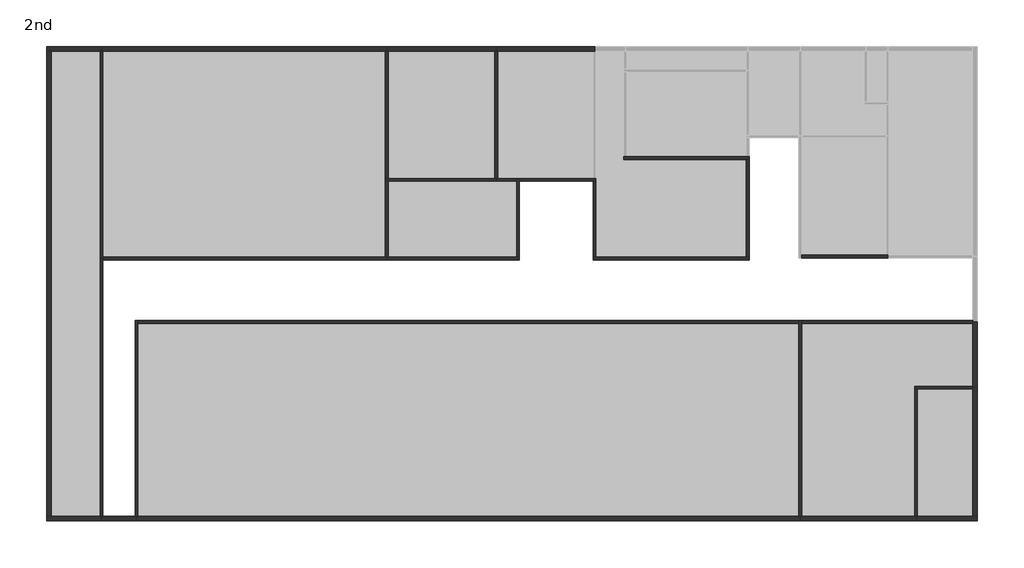
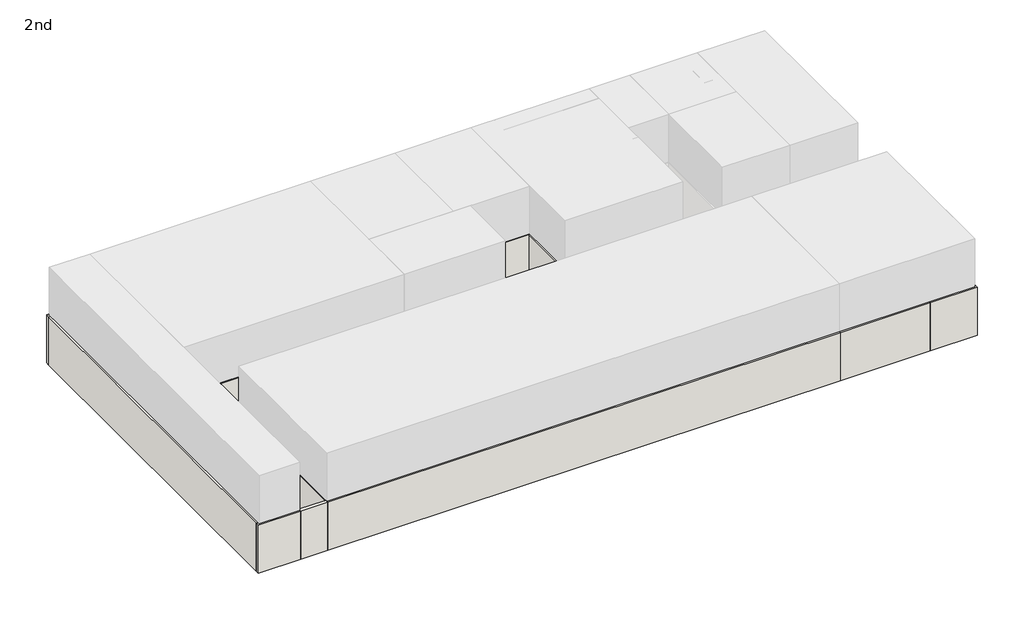
# One storey, part 1 of 2: 56 walls.
"""IFC4 building model written with IfcOpenShell, lengths in millimetres."""

from ifc_helpers import new_model, si_unit, frame, origin, place, context, project, spatial, polyline, outline, extrude, faceted_brep, element, save

model = new_model("IFC4")

# Units and contexts
model_context = context("Model", 3, world=origin())
ifc_project = project(units=[si_unit("LENGTHUNIT", "METRE", prefix="MILLI")], contexts=[model_context])

# Site, building, storey
site = spatial("IfcSite", under=ifc_project)
building = spatial("IfcBuilding", under=site)
storey = spatial("IfcBuildingStorey", under=building, Name="2nd", Elevation=14000.0)

# Walls
placement = place(None, origin())
element("IfcWall", 1, ObjectType="Wall-Ext_215Bwk", at=placement, inside=storey, context=model_context, shape_type="Brep", body=[
    faceted_brep([(11750.0, 151142.5, 14000.0), (42100.0, 151142.5, 14000.0), (42100.0, 151142.5, 17000.0), (11750.0, 151142.5, 17000.0), (11750.0, 151357.5, 14000.0), (11750.0, 151357.5, 17000.0), (11812.5, 151357.5, 17000.0), (42037.5, 151357.5, 17000.0), (42100.0, 151357.5, 17000.0), (42100.0, 151357.5, 14000.0), (42037.5, 151357.5, 14000.0), (11812.5, 151357.5, 14000.0)], [[[0, 1, 2, 3]], [[4, 5, 6, 7, 8, 9, 10, 11]], [[1, 0, 4, 11, 10, 9]], [[2, 1, 9, 8]], [[3, 2, 8, 7, 6, 5]], [[0, 3, 5, 4]]]),
])
element("IfcWall", 2, ObjectType="Wall-Ext_215Bwk", at=placement, inside=storey, context=model_context, shape_type="Brep", body=[
    faceted_brep([(23200.0, 172857.5, 14000.0), (10150.0, 172857.5, 14000.0), (10150.0, 172857.5, 17000.0), (23200.0, 172857.5, 17000.0), (23200.0, 172642.5, 14000.0), (23200.0, 172642.5, 17000.0), (23137.5, 172642.5, 17000.0), (10212.5, 172642.5, 17000.0), (10150.0, 172642.5, 17000.0), (10150.0, 172642.5, 14000.0), (10212.5, 172642.5, 14000.0), (23137.5, 172642.5, 14000.0)], [[[0, 1, 2, 3]], [[4, 5, 6, 7, 8, 9, 10, 11]], [[1, 0, 4, 11, 10, 9]], [[2, 1, 9, 8]], [[3, 2, 8, 7, 6, 5]], [[0, 3, 5, 4]]]),
])
element("IfcWall", 3, ObjectType="Wall-Ext_215Bwk", at=placement, inside=storey, context=model_context, shape_type="Brep", body=[
    faceted_brep([(28200.0, 172857.5, 14000.0), (23200.0, 172857.5, 14000.0), (23200.0, 172857.5, 17000.0), (28200.0, 172857.5, 17000.0), (28200.0, 172642.5, 14000.0), (28200.0, 172642.5, 17000.0), (28137.5, 172642.5, 17000.0), (23262.5, 172642.5, 17000.0), (23200.0, 172642.5, 17000.0), (23200.0, 172642.5, 14000.0), (23262.5, 172642.5, 14000.0), (28137.5, 172642.5, 14000.0)], [[[0, 1, 2, 3]], [[4, 5, 6, 7, 8, 9, 10, 11]], [[1, 0, 4, 11, 10, 9]], [[2, 1, 9, 8]], [[3, 2, 8, 7, 6, 5]], [[0, 3, 5, 4]]]),
])
element("IfcWall", 4, ObjectType="Wall-Ext_215Bwk", at=placement, inside=storey, context=model_context, shape_type="SweptSolid", body=[
    extrude(outline(polyline([(7642.5, 151357.5), (7642.5, 172642.5), (7857.5, 172642.5), (7857.5, 151357.5), (7642.5, 151357.5)])), frame((0.0, 0.0, 14000.0), z_axis=(0.0, 0.0, 1.0), x_axis=(1.0, 0.0, 0.0)), (0.0, 0.0, 1.0), 3000.0),
])
element("IfcWall", 5, ObjectType="Wall-Ext_215Bwk", at=placement, inside=storey, context=model_context, shape_type="Brep", body=[
    faceted_brep([(7642.5, 151142.5, 14000.0), (10150.0, 151142.5, 14000.0), (10150.0, 151142.5, 17000.0), (7642.5, 151142.5, 17000.0), (7642.5, 151357.5, 14000.0), (7642.5, 151357.5, 17000.0), (7857.5, 151357.5, 17000.0), (10087.5, 151357.5, 17000.0), (10150.0, 151357.5, 17000.0), (10150.0, 151357.5, 14000.0), (10087.5, 151357.5, 14000.0), (7857.5, 151357.5, 14000.0)], [[[0, 1, 2, 3]], [[4, 5, 6, 7, 8, 9, 10, 11]], [[1, 0, 4, 11, 10, 9]], [[2, 1, 9, 8]], [[3, 2, 8, 7, 6, 5]], [[0, 3, 5, 4]]]),
])
element("IfcWall", 6, ObjectType="Wall-Ext_215Bwk", at=placement, inside=storey, context=model_context, shape_type="Brep", body=[
    faceted_brep([(10150.0, 172857.5, 14000.0), (7642.5, 172857.5, 14000.0), (7642.5, 172857.5, 17000.0), (10150.0, 172857.5, 17000.0), (10150.0, 172642.5, 14000.0), (10150.0, 172642.5, 17000.0), (10087.5, 172642.5, 17000.0), (7857.5, 172642.5, 17000.0), (7642.5, 172642.5, 17000.0), (7642.5, 172642.5, 14000.0), (7857.5, 172642.5, 14000.0), (10087.5, 172642.5, 14000.0)], [[[0, 1, 2, 3]], [[4, 5, 6, 7, 8, 9, 10, 11]], [[1, 0, 4, 11, 10, 9]], [[3, 2, 8, 7, 6, 5]], [[0, 3, 5, 4]], [[2, 1, 9, 8]]]),
])
element("IfcWall", 7, ObjectType="Wall-Ext_215Bwk", at=placement, inside=storey, context=model_context, shape_type="Brep", body=[
    faceted_brep([(32700.0, 172857.5, 14000.0), (28200.0, 172857.5, 14000.0), (28200.0, 172857.5, 17000.0), (32700.0, 172857.5, 17000.0), (32700.0, 172642.5, 14000.0), (32700.0, 172642.5, 17000.0), (32637.5, 172642.5, 17000.0), (28262.5, 172642.5, 17000.0), (28200.0, 172642.5, 17000.0), (28200.0, 172642.5, 14000.0), (28262.5, 172642.5, 14000.0), (32637.5, 172642.5, 14000.0)], [[[0, 1, 2, 3]], [[4, 5, 6, 7, 8, 9, 10, 11]], [[1, 0, 4, 11, 10, 9]], [[2, 1, 9, 8]], [[3, 2, 8, 7, 6, 5]], [[0, 3, 5, 4]]]),
])
element("IfcWall", 8, ObjectType="Wall-Ext_215Bwk", at=placement, inside=storey, context=model_context, shape_type="Brep", body=[
    faceted_brep([(50207.5, 157250.0, 14000.0), (50207.5, 160250.0, 14000.0), (50207.5, 160250.0, 17000.0), (50207.5, 157250.0, 17000.0), (49992.5, 157250.0, 14000.0), (49992.5, 157250.0, 17000.0), (49992.5, 157312.5, 17000.0), (49992.5, 160187.5, 17000.0), (49992.5, 160250.0, 17000.0), (49992.5, 160250.0, 14000.0), (49992.5, 160187.5, 14000.0), (49992.5, 157312.5, 14000.0)], [[[0, 1, 2, 3]], [[4, 5, 6, 7, 8, 9, 10, 11]], [[1, 0, 4, 11, 10, 9]], [[2, 1, 9, 8]], [[3, 2, 8, 7, 6, 5]], [[0, 3, 5, 4]]]),
])
element("IfcWall", 9, ObjectType="Wall-Ext_215Bwk", at=placement, inside=storey, context=model_context, shape_type="Brep", body=[
    faceted_brep([(42100.0, 151142.5, 14000.0), (47400.0, 151142.5, 14000.0), (47400.0, 151142.5, 17000.0), (42100.0, 151142.5, 17000.0), (42100.0, 151357.5, 14000.0), (42100.0, 151357.5, 17000.0), (42162.5, 151357.5, 17000.0), (47337.5, 151357.5, 17000.0), (47400.0, 151357.5, 17000.0), (47400.0, 151357.5, 14000.0), (47337.5, 151357.5, 14000.0), (42162.5, 151357.5, 14000.0)], [[[0, 1, 2, 3]], [[4, 5, 6, 7, 8, 9, 10, 11]], [[1, 0, 4, 11, 10, 9]], [[2, 1, 9, 8]], [[3, 2, 8, 7, 6, 5]], [[0, 3, 5, 4]]]),
])
element("IfcWall", 10, ObjectType="Wall-Ext_215Bwk", at=placement, inside=storey, context=model_context, shape_type="Brep", body=[
    faceted_brep([(50207.5, 151357.5, 14000.0), (50207.5, 157250.0, 14000.0), (50207.5, 157250.0, 17000.0), (50207.5, 151357.5, 17000.0), (49992.5, 151357.5, 14000.0), (49992.5, 151357.5, 17000.0), (49992.5, 157187.5, 17000.0), (49992.5, 157250.0, 17000.0), (49992.5, 157250.0, 14000.0), (49992.5, 157187.5, 14000.0)], [[[0, 1, 2, 3]], [[4, 5, 6, 7, 8, 9]], [[1, 0, 4, 9, 8]], [[2, 1, 8, 7]], [[3, 2, 7, 6, 5]], [[0, 3, 5, 4]]]),
])
element("IfcWall", 11, ObjectType="Wall-Ext_215Bwk", at=placement, inside=storey, context=model_context, shape_type="Brep", body=[
    faceted_brep([(47400.0, 151142.5, 14000.0), (50207.5, 151142.5, 14000.0), (50207.5, 151142.5, 17000.0), (47400.0, 151142.5, 17000.0), (47400.0, 151357.5, 14000.0), (47400.0, 151357.5, 17000.0), (47462.5, 151357.5, 17000.0), (49992.5, 151357.5, 17000.0), (50207.5, 151357.5, 17000.0), (50207.5, 151357.5, 14000.0), (49992.5, 151357.5, 14000.0), (47462.5, 151357.5, 14000.0)], [[[0, 1, 2, 3]], [[4, 5, 6, 7, 8, 9, 10, 11]], [[1, 0, 4, 11, 10, 9]], [[3, 2, 8, 7, 6, 5]], [[0, 3, 5, 4]], [[2, 1, 9, 8]]]),
])
element("IfcWall", 12, ObjectType="Wall-Ext_215Bwk", at=placement, inside=storey, context=model_context, shape_type="Brep", body=[
    faceted_brep([(10150.0, 151142.5, 14000.0), (11750.0, 151142.5, 14000.0), (11750.0, 151142.5, 17000.0), (10150.0, 151142.5, 17000.0), (10150.0, 151357.5, 14000.0), (10150.0, 151357.5, 17000.0), (10212.5, 151357.5, 17000.0), (11687.5, 151357.5, 17000.0), (11750.0, 151357.5, 17000.0), (11750.0, 151357.5, 14000.0), (11687.5, 151357.5, 14000.0), (10212.5, 151357.5, 14000.0)], [[[0, 1, 2, 3]], [[4, 5, 6, 7, 8, 9, 10, 11]], [[1, 0, 4, 11, 10, 9]], [[2, 1, 9, 8]], [[3, 2, 8, 7, 6, 5]], [[0, 3, 5, 4]]]),
])
element("IfcWall", 13, ObjectType="Wall-Int_12P-100Blk-12P", at=placement, inside=storey, context=model_context, shape_type="SweptSolid", body=[
    extrude(outline(polyline([(11812.5, 160312.5), (42037.5, 160312.5), (42037.5, 160187.5), (11812.5, 160187.5), (11812.5, 160312.5)])), frame((0.0, 0.0, 14000.0), z_axis=(0.0, 0.0, 1.0), x_axis=(1.0, 0.0, 0.0)), (0.0, 0.0, 1.0), 3000.0),
])
element("IfcWall", 14, ObjectType="Wall-Int_12P-100Blk-12P", at=placement, inside=storey, context=model_context, shape_type="Brep", body=[
    faceted_brep([(11687.5, 160312.5, 14000.0), (11687.5, 151357.5, 14000.0), (11687.5, 151357.5, 17000.0), (11687.5, 160312.5, 17000.0), (11812.5, 160312.5, 14000.0), (11812.5, 160312.5, 17000.0), (11812.5, 160187.5, 17000.0), (11812.5, 151357.5, 17000.0), (11812.5, 151357.5, 14000.0), (11812.5, 160187.5, 14000.0), (11750.0, 151357.5, 14000.0), (11750.0, 151357.5, 17000.0)], [[[0, 1, 2, 3]], [[4, 5, 6, 7, 8, 9]], [[1, 0, 4, 9, 8, 10]], [[3, 2, 11, 7, 6, 5]], [[0, 3, 5, 4]], [[2, 1, 10, 8, 7, 11]]]),
])
element("IfcWall", 15, ObjectType="Wall-Int_12P-100Blk-12P", at=placement, inside=storey, context=model_context, shape_type="Brep", body=[
    faceted_brep([(42162.5, 151357.5, 14000.0), (42162.5, 160187.5, 14000.0), (42162.5, 160312.5, 14000.0), (42162.5, 160312.5, 17000.0), (42162.5, 160187.5, 17000.0), (42162.5, 151357.5, 17000.0), (42037.5, 151357.5, 14000.0), (42037.5, 151357.5, 17000.0), (42037.5, 160187.5, 17000.0), (42037.5, 160312.5, 17000.0), (42037.5, 160312.5, 14000.0), (42037.5, 160187.5, 14000.0), (42100.0, 151357.5, 14000.0), (42100.0, 151357.5, 17000.0)], [[[0, 1, 2, 3, 4, 5]], [[6, 7, 8, 9, 10, 11]], [[2, 1, 0, 12, 6, 11, 10]], [[5, 4, 3, 9, 8, 7, 13]], [[3, 2, 10, 9]], [[0, 5, 13, 7, 6, 12]]]),
])
element("IfcWall", 16, ObjectType="Wall-Int_12P-100Blk-12P", at=placement, inside=storey, context=model_context, shape_type="Brep", body=[
    faceted_brep([(10087.5, 172642.5, 14000.0), (10087.5, 163150.0, 14000.0), (10087.5, 163150.0, 17000.0), (10087.5, 172642.5, 17000.0), (10212.5, 172642.5, 14000.0), (10212.5, 172642.5, 17000.0), (10212.5, 163212.5, 17000.0), (10212.5, 163150.0, 17000.0), (10212.5, 163150.0, 14000.0), (10212.5, 163212.5, 14000.0), (10150.0, 172642.5, 14000.0), (10150.0, 172642.5, 17000.0)], [[[0, 1, 2, 3]], [[4, 5, 6, 7, 8, 9]], [[1, 0, 10, 4, 9, 8]], [[2, 1, 8, 7]], [[3, 2, 7, 6, 5, 11]], [[0, 3, 11, 5, 4, 10]]]),
])
element("IfcWall", 17, ObjectType="Wall-Int_12P-100Blk-12P", at=placement, inside=storey, context=model_context, shape_type="Brep", body=[
    faceted_brep([(10212.5, 163087.5, 14000.0), (23200.0, 163087.5, 14000.0), (23200.0, 163087.5, 17000.0), (10212.5, 163087.5, 17000.0), (10212.5, 163212.5, 14000.0), (10212.5, 163212.5, 17000.0), (23137.5, 163212.5, 17000.0), (23200.0, 163212.5, 17000.0), (23200.0, 163212.5, 14000.0), (23137.5, 163212.5, 14000.0), (10212.5, 163150.0, 14000.0), (10212.5, 163150.0, 17000.0)], [[[0, 1, 2, 3]], [[4, 5, 6, 7, 8, 9]], [[1, 0, 10, 4, 9, 8]], [[2, 1, 8, 7]], [[3, 2, 7, 6, 5, 11]], [[0, 3, 11, 5, 4, 10]]]),
])
element("IfcWall", 18, ObjectType="Wall-Int_12P-100Blk-12P", at=placement, inside=storey, context=model_context, shape_type="Brep", body=[
    faceted_brep([(23262.5, 163212.5, 14000.0), (23262.5, 166687.5, 14000.0), (23262.5, 166687.5, 17000.0), (23262.5, 163212.5, 17000.0), (23137.5, 163212.5, 14000.0), (23137.5, 163212.5, 17000.0), (23137.5, 166687.5, 17000.0), (23137.5, 166687.5, 14000.0), (23200.0, 163212.5, 14000.0), (23200.0, 163212.5, 17000.0)], [[[0, 1, 2, 3]], [[4, 5, 6, 7]], [[1, 0, 8, 4, 7]], [[3, 2, 6, 5, 9]], [[0, 3, 9, 5, 4, 8]], [[2, 1, 7, 6]]]),
])
element("IfcWall", 19, ObjectType="Wall-Int_12P-100Blk-12P", at=placement, inside=storey, context=model_context, shape_type="Brep", body=[
    faceted_brep([(23262.5, 166812.5, 14000.0), (23262.5, 172642.5, 14000.0), (23262.5, 172642.5, 17000.0), (23262.5, 166812.5, 17000.0), (23137.5, 166812.5, 14000.0), (23137.5, 166812.5, 17000.0), (23137.5, 172642.5, 17000.0), (23137.5, 172642.5, 14000.0), (23200.0, 172642.5, 14000.0), (23200.0, 172642.5, 17000.0)], [[[0, 1, 2, 3]], [[4, 5, 6, 7]], [[1, 0, 4, 7, 8]], [[3, 2, 9, 6, 5]], [[0, 3, 5, 4]], [[2, 1, 8, 7, 6, 9]]]),
])
element("IfcWall", 20, ObjectType="Wall-Int_12P-100Blk-12P", at=placement, inside=storey, context=model_context, shape_type="Brep", body=[
    faceted_brep([(23137.5, 172642.5, 14000.0), (23137.5, 166812.5, 14000.0), (23137.5, 166812.5, 17000.0), (23137.5, 172642.5, 17000.0), (23262.5, 172642.5, 14000.0), (23262.5, 172642.5, 17000.0), (23262.5, 166812.5, 17000.0), (23262.5, 166812.5, 14000.0), (23200.0, 172642.5, 14000.0), (23200.0, 172642.5, 17000.0)], [[[0, 1, 2, 3]], [[4, 5, 6, 7]], [[1, 0, 8, 4, 7]], [[3, 2, 6, 5, 9]], [[2, 1, 7, 6]], [[0, 3, 9, 5, 4, 8]]]),
])
element("IfcWall", 21, ObjectType="Wall-Int_12P-100Blk-12P", at=placement, inside=storey, context=model_context, shape_type="Brep", body=[
    faceted_brep([(23137.5, 166687.5, 14000.0), (23262.5, 166687.5, 14000.0), (28200.0, 166687.5, 14000.0), (28200.0, 166687.5, 17000.0), (23262.5, 166687.5, 17000.0), (23137.5, 166687.5, 17000.0), (23137.5, 166812.5, 14000.0), (23137.5, 166812.5, 17000.0), (23262.5, 166812.5, 17000.0), (28137.5, 166812.5, 17000.0), (28200.0, 166812.5, 17000.0), (28200.0, 166812.5, 14000.0), (28137.5, 166812.5, 14000.0), (23262.5, 166812.5, 14000.0)], [[[0, 1, 2, 3, 4, 5]], [[6, 7, 8, 9, 10, 11, 12, 13]], [[2, 1, 0, 6, 13, 12, 11]], [[3, 2, 11, 10]], [[5, 4, 3, 10, 9, 8, 7]], [[0, 5, 7, 6]]]),
])
element("IfcWall", 22, ObjectType="Wall-Int_12P-100Blk-12P", at=placement, inside=storey, context=model_context, shape_type="Brep", body=[
    faceted_brep([(28262.5, 166812.5, 14000.0), (28262.5, 172642.5, 14000.0), (28262.5, 172642.5, 17000.0), (28262.5, 166812.5, 17000.0), (28137.5, 166812.5, 14000.0), (28137.5, 166812.5, 17000.0), (28137.5, 172642.5, 17000.0), (28137.5, 172642.5, 14000.0), (28200.0, 166812.5, 14000.0), (28200.0, 172642.5, 14000.0), (28200.0, 172642.5, 17000.0), (28200.0, 166812.5, 17000.0)], [[[0, 1, 2, 3]], [[4, 5, 6, 7]], [[1, 0, 8, 4, 7, 9]], [[3, 2, 10, 6, 5, 11]], [[0, 3, 11, 5, 4, 8]], [[2, 1, 9, 7, 6, 10]]]),
])
element("IfcWall", 23, ObjectType="Wall-Int_12P-100Blk-12P", at=placement, inside=storey, context=model_context, shape_type="Brep", body=[
    faceted_brep([(42162.5, 163187.5, 14000.0), (46100.0, 163187.5, 14000.0), (46100.0, 163187.5, 17000.0), (42162.5, 163187.5, 17000.0), (42162.5, 163312.5, 14000.0), (42162.5, 163312.5, 17000.0), (46037.5, 163312.5, 17000.0), (46100.0, 163312.5, 17000.0), (46100.0, 163312.5, 14000.0), (46037.5, 163312.5, 14000.0)], [[[0, 1, 2, 3]], [[4, 5, 6, 7, 8, 9]], [[1, 0, 4, 9, 8]], [[2, 1, 8, 7]], [[3, 2, 7, 6, 5]], [[0, 3, 5, 4]]]),
])
element("IfcWall", 24, ObjectType="Wall-Int_12P-100Blk-12P", at=placement, inside=storey, context=model_context, shape_type="Brep", body=[
    faceted_brep([(10212.5, 163150.0, 14000.0), (10212.5, 163212.5, 14000.0), (10212.5, 172642.5, 14000.0), (10212.5, 172642.5, 17000.0), (10212.5, 163212.5, 17000.0), (10212.5, 163150.0, 17000.0), (10087.5, 163150.0, 14000.0), (10087.5, 163150.0, 17000.0), (10087.5, 172642.5, 17000.0), (10087.5, 172642.5, 14000.0), (10150.0, 172642.5, 14000.0), (10150.0, 172642.5, 17000.0)], [[[0, 1, 2, 3, 4, 5]], [[6, 7, 8, 9]], [[2, 1, 0, 6, 9, 10]], [[5, 4, 3, 11, 8, 7]], [[0, 5, 7, 6]], [[3, 2, 10, 9, 8, 11]]]),
])
element("IfcWall", 25, ObjectType="Wall-Int_12P-100Blk-12P", at=placement, inside=storey, context=model_context, shape_type="Brep", body=[
    faceted_brep([(10212.5, 151357.5, 14000.0), (10212.5, 163087.5, 14000.0), (10212.5, 163150.0, 14000.0), (10212.5, 163150.0, 17000.0), (10212.5, 163087.5, 17000.0), (10212.5, 151357.5, 17000.0), (10087.5, 151357.5, 14000.0), (10087.5, 151357.5, 17000.0), (10087.5, 163150.0, 17000.0), (10087.5, 163150.0, 14000.0), (10150.0, 151357.5, 14000.0), (10150.0, 151357.5, 17000.0)], [[[0, 1, 2, 3, 4, 5]], [[6, 7, 8, 9]], [[2, 1, 0, 10, 6, 9]], [[3, 2, 9, 8]], [[5, 4, 3, 8, 7, 11]], [[0, 5, 11, 7, 6, 10]]]),
])
element("IfcWall", 26, ObjectType="Wall-Int_12P-100Blk-12P", at=placement, inside=storey, context=model_context, shape_type="Brep", body=[
    faceted_brep([(28137.5, 172642.5, 14000.0), (28137.5, 166812.5, 14000.0), (28137.5, 166812.5, 17000.0), (28137.5, 172642.5, 17000.0), (28262.5, 172642.5, 14000.0), (28262.5, 172642.5, 17000.0), (28262.5, 166812.5, 17000.0), (28262.5, 166812.5, 14000.0), (28200.0, 172642.5, 14000.0), (28200.0, 166812.5, 14000.0), (28200.0, 166812.5, 17000.0), (28200.0, 172642.5, 17000.0)], [[[0, 1, 2, 3]], [[4, 5, 6, 7]], [[1, 0, 8, 4, 7, 9]], [[3, 2, 10, 6, 5, 11]], [[2, 1, 9, 7, 6, 10]], [[0, 3, 11, 5, 4, 8]]]),
])
element("IfcWall", 27, ObjectType="Wall-Int_12P-100Blk-12P", at=placement, inside=storey, context=model_context, shape_type="Brep", body=[
    faceted_brep([(28200.0, 166687.5, 14000.0), (29137.5, 166687.5, 14000.0), (29137.5, 166687.5, 17000.0), (28200.0, 166687.5, 17000.0), (28200.0, 166812.5, 14000.0), (28200.0, 166812.5, 17000.0), (28262.5, 166812.5, 17000.0), (29137.5, 166812.5, 17000.0), (29137.5, 166812.5, 14000.0), (28262.5, 166812.5, 14000.0)], [[[0, 1, 2, 3]], [[4, 5, 6, 7, 8, 9]], [[1, 0, 4, 9, 8]], [[3, 2, 7, 6, 5]], [[0, 3, 5, 4]], [[2, 1, 8, 7]]]),
])
element("IfcWall", 28, ObjectType="Wall-Int_12P-100Blk-12P", at=placement, inside=storey, context=model_context, shape_type="Brep", body=[
    faceted_brep([(29262.5, 166687.5, 14000.0), (32637.5, 166687.5, 14000.0), (32762.5, 166687.5, 14000.0), (32762.5, 166687.5, 17000.0), (32637.5, 166687.5, 17000.0), (29262.5, 166687.5, 17000.0), (29262.5, 166812.5, 14000.0), (29262.5, 166812.5, 17000.0), (32637.5, 166812.5, 17000.0), (32762.5, 166812.5, 17000.0), (32762.5, 166812.5, 14000.0), (32637.5, 166812.5, 14000.0)], [[[0, 1, 2, 3, 4, 5]], [[6, 7, 8, 9, 10, 11]], [[2, 1, 0, 6, 11, 10]], [[5, 4, 3, 9, 8, 7]], [[3, 2, 10, 9]], [[0, 5, 7, 6]]]),
])
element("IfcWall", 29, ObjectType="Wall-Int_12P-100Blk-12P", at=placement, inside=storey, context=model_context, shape_type="Brep", body=[
    faceted_brep([(23137.5, 166687.5, 14000.0), (23137.5, 163212.5, 14000.0), (23137.5, 163212.5, 17000.0), (23137.5, 166687.5, 17000.0), (23262.5, 166687.5, 14000.0), (23262.5, 166687.5, 17000.0), (23262.5, 163212.5, 17000.0), (23262.5, 163212.5, 14000.0), (23200.0, 163212.5, 14000.0), (23200.0, 163212.5, 17000.0)], [[[0, 1, 2, 3]], [[4, 5, 6, 7]], [[1, 0, 4, 7, 8]], [[3, 2, 9, 6, 5]], [[2, 1, 8, 7, 6, 9]], [[0, 3, 5, 4]]]),
])
element("IfcWall", 30, ObjectType="Wall-Int_12P-100Blk-12P", at=placement, inside=storey, context=model_context, shape_type="Brep", body=[
    faceted_brep([(23200.0, 163087.5, 14000.0), (29262.5, 163087.5, 14000.0), (29262.5, 163087.5, 17000.0), (23200.0, 163087.5, 17000.0), (23200.0, 163212.5, 14000.0), (23200.0, 163212.5, 17000.0), (23262.5, 163212.5, 17000.0), (29137.5, 163212.5, 17000.0), (29262.5, 163212.5, 17000.0), (29262.5, 163212.5, 14000.0), (29137.5, 163212.5, 14000.0), (23262.5, 163212.5, 14000.0)], [[[0, 1, 2, 3]], [[4, 5, 6, 7, 8, 9, 10, 11]], [[1, 0, 4, 11, 10, 9]], [[3, 2, 8, 7, 6, 5]], [[0, 3, 5, 4]], [[2, 1, 9, 8]]]),
])
element("IfcWall", 31, ObjectType="Wall-Int_12P-100Blk-12P", at=placement, inside=storey, context=model_context, shape_type="Brep", body=[
    faceted_brep([(29262.5, 163212.5, 14000.0), (29262.5, 166687.5, 14000.0), (29262.5, 166812.5, 14000.0), (29262.5, 166812.5, 17000.0), (29262.5, 166687.5, 17000.0), (29262.5, 163212.5, 17000.0), (29137.5, 163212.5, 14000.0), (29137.5, 163212.5, 17000.0), (29137.5, 166687.5, 17000.0), (29137.5, 166812.5, 17000.0), (29137.5, 166812.5, 14000.0), (29137.5, 166687.5, 14000.0)], [[[0, 1, 2, 3, 4, 5]], [[6, 7, 8, 9, 10, 11]], [[2, 1, 0, 6, 11, 10]], [[5, 4, 3, 9, 8, 7]], [[3, 2, 10, 9]], [[0, 5, 7, 6]]]),
])
element("IfcWall", 32, ObjectType="Wall-Int_12P-100Blk-12P", at=placement, inside=storey, context=model_context, shape_type="Brep", body=[
    faceted_brep([(29137.5, 166812.5, 14000.0), (28262.5, 166812.5, 14000.0), (28200.0, 166812.5, 14000.0), (28200.0, 166812.5, 17000.0), (28262.5, 166812.5, 17000.0), (29137.5, 166812.5, 17000.0), (29137.5, 166687.5, 14000.0), (29137.5, 166687.5, 17000.0), (28200.0, 166687.5, 17000.0), (28200.0, 166687.5, 14000.0)], [[[0, 1, 2, 3, 4, 5]], [[6, 7, 8, 9]], [[2, 1, 0, 6, 9]], [[3, 2, 9, 8]], [[5, 4, 3, 8, 7]], [[0, 5, 7, 6]]]),
])
element("IfcWall", 33, ObjectType="Wall-Int_12P-100Blk-12P", at=placement, inside=storey, context=model_context, shape_type="Brep", body=[
    faceted_brep([(28200.0, 166812.5, 14000.0), (28137.5, 166812.5, 14000.0), (23262.5, 166812.5, 14000.0), (23137.5, 166812.5, 14000.0), (23137.5, 166812.5, 17000.0), (23262.5, 166812.5, 17000.0), (28137.5, 166812.5, 17000.0), (28200.0, 166812.5, 17000.0), (28200.0, 166687.5, 14000.0), (28200.0, 166687.5, 17000.0), (23262.5, 166687.5, 17000.0), (23137.5, 166687.5, 17000.0), (23137.5, 166687.5, 14000.0), (23262.5, 166687.5, 14000.0)], [[[0, 1, 2, 3, 4, 5, 6, 7]], [[8, 9, 10, 11, 12, 13]], [[3, 2, 1, 0, 8, 13, 12]], [[7, 6, 5, 4, 11, 10, 9]], [[0, 7, 9, 8]], [[4, 3, 12, 11]]]),
])
element("IfcWall", 34, ObjectType="Wall-Int_12P-100Blk-12P", at=placement, inside=storey, context=model_context, shape_type="SweptSolid", body=[
    extrude(outline(polyline([(32637.5, 163212.5), (32637.5, 166687.5), (32762.5, 166687.5), (32762.5, 163212.5), (32637.5, 163212.5)])), frame((0.0, 0.0, 14000.0), z_axis=(0.0, 0.0, 1.0), x_axis=(1.0, 0.0, 0.0)), (0.0, 0.0, 1.0), 3000.0),
])
element("IfcWall", 35, ObjectType="Wall-Int_12P-100Blk-12P", at=placement, inside=storey, context=model_context, shape_type="Brep", body=[
    faceted_brep([(32637.5, 163087.5, 14000.0), (39762.5, 163087.5, 14000.0), (39762.5, 163087.5, 17000.0), (32637.5, 163087.5, 17000.0), (32637.5, 163212.5, 14000.0), (32637.5, 163212.5, 17000.0), (32762.5, 163212.5, 17000.0), (39637.5, 163212.5, 17000.0), (39762.5, 163212.5, 17000.0), (39762.5, 163212.5, 14000.0), (39637.5, 163212.5, 14000.0), (32762.5, 163212.5, 14000.0)], [[[0, 1, 2, 3]], [[4, 5, 6, 7, 8, 9, 10, 11]], [[1, 0, 4, 11, 10, 9]], [[3, 2, 8, 7, 6, 5]], [[0, 3, 5, 4]], [[2, 1, 9, 8]]]),
])
element("IfcWall", 36, ObjectType="Wall-Int_12P-100Blk-12P", at=placement, inside=storey, context=model_context, shape_type="SweptSolid", body=[
    extrude(outline(polyline([(39762.5, 167687.5), (39762.5, 163212.5), (39637.5, 163212.5), (39637.5, 167687.5), (39762.5, 167687.5)])), frame((0.0, 0.0, 14000.0), z_axis=(0.0, 0.0, 1.0), x_axis=(1.0, 0.0, 0.0)), (0.0, 0.0, 1.0), 3000.0),
])
element("IfcWall", 37, ObjectType="Wall-Int_12P-100Blk-12P", at=placement, inside=storey, context=model_context, shape_type="Brep", body=[
    faceted_brep([(39762.5, 167812.5, 14000.0), (39637.5, 167812.5, 14000.0), (34162.5, 167812.5, 14000.0), (34037.5, 167812.5, 14000.0), (34037.5, 167812.5, 17000.0), (34162.5, 167812.5, 17000.0), (39637.5, 167812.5, 17000.0), (39762.5, 167812.5, 17000.0), (39762.5, 167687.5, 14000.0), (39762.5, 167687.5, 17000.0), (39637.5, 167687.5, 17000.0), (34037.5, 167687.5, 17000.0), (34037.5, 167687.5, 14000.0), (39637.5, 167687.5, 14000.0)], [[[0, 1, 2, 3, 4, 5, 6, 7]], [[8, 9, 10, 11, 12, 13]], [[3, 2, 1, 0, 8, 13, 12]], [[7, 6, 5, 4, 11, 10, 9]], [[4, 3, 12, 11]], [[0, 7, 9, 8]]]),
])
element("IfcWall", 38, ObjectType="Wall-Int_12P-100Blk-12P", at=placement, inside=storey, context=model_context, shape_type="Brep", body=[
    faceted_brep([(34037.5, 167687.5, 14000.0), (39637.5, 167687.5, 14000.0), (39762.5, 167687.5, 14000.0), (39762.5, 167687.5, 17000.0), (39637.5, 167687.5, 17000.0), (34037.5, 167687.5, 17000.0), (34037.5, 167812.5, 14000.0), (34037.5, 167812.5, 17000.0), (34162.5, 167812.5, 17000.0), (39637.5, 167812.5, 17000.0), (39762.5, 167812.5, 17000.0), (39762.5, 167812.5, 14000.0), (39637.5, 167812.5, 14000.0), (34162.5, 167812.5, 14000.0)], [[[0, 1, 2, 3, 4, 5]], [[6, 7, 8, 9, 10, 11, 12, 13]], [[2, 1, 0, 6, 13, 12, 11]], [[5, 4, 3, 10, 9, 8, 7]], [[0, 5, 7, 6]], [[3, 2, 11, 10]]]),
])
element("IfcWall", 39, ObjectType="Wall-Int_12P-100Blk-12P", at=placement, inside=storey, context=model_context, shape_type="Brep", body=[
    faceted_brep([(42037.5, 160312.5, 14000.0), (42037.5, 160187.5, 14000.0), (42037.5, 151357.5, 14000.0), (42037.5, 151357.5, 17000.0), (42037.5, 160187.5, 17000.0), (42037.5, 160312.5, 17000.0), (42162.5, 160312.5, 14000.0), (42162.5, 160312.5, 17000.0), (42162.5, 160187.5, 17000.0), (42162.5, 151357.5, 17000.0), (42162.5, 151357.5, 14000.0), (42162.5, 160187.5, 14000.0), (42100.0, 151357.5, 14000.0), (42100.0, 151357.5, 17000.0)], [[[0, 1, 2, 3, 4, 5]], [[6, 7, 8, 9, 10, 11]], [[2, 1, 0, 6, 11, 10, 12]], [[5, 4, 3, 13, 9, 8, 7]], [[0, 5, 7, 6]], [[3, 2, 12, 10, 9, 13]]]),
])
element("IfcWall", 40, ObjectType="Wall-Int_12P-100Blk-12P", at=placement, inside=storey, context=model_context, shape_type="Brep", body=[
    faceted_brep([(47462.5, 151357.5, 14000.0), (47462.5, 157187.5, 14000.0), (47462.5, 157187.5, 17000.0), (47462.5, 151357.5, 17000.0), (47337.5, 151357.5, 14000.0), (47337.5, 151357.5, 17000.0), (47337.5, 157187.5, 17000.0), (47337.5, 157187.5, 14000.0), (47400.0, 151357.5, 14000.0), (47400.0, 151357.5, 17000.0)], [[[0, 1, 2, 3]], [[4, 5, 6, 7]], [[1, 0, 8, 4, 7]], [[3, 2, 6, 5, 9]], [[2, 1, 7, 6]], [[0, 3, 9, 5, 4, 8]]]),
])
element("IfcWall", 41, ObjectType="Wall-Int_12P-100Blk-12P", at=placement, inside=storey, context=model_context, shape_type="Brep", body=[
    faceted_brep([(47337.5, 157187.5, 14000.0), (47462.5, 157187.5, 14000.0), (49992.5, 157187.5, 14000.0), (49992.5, 157187.5, 17000.0), (47462.5, 157187.5, 17000.0), (47337.5, 157187.5, 17000.0), (47337.5, 157312.5, 14000.0), (47337.5, 157312.5, 17000.0), (49992.5, 157312.5, 17000.0), (49992.5, 157312.5, 14000.0), (49992.5, 157250.0, 14000.0), (49992.5, 157250.0, 17000.0)], [[[0, 1, 2, 3, 4, 5]], [[6, 7, 8, 9]], [[2, 1, 0, 6, 9, 10]], [[5, 4, 3, 11, 8, 7]], [[0, 5, 7, 6]], [[3, 2, 10, 9, 8, 11]]]),
])
element("IfcWall", 42, ObjectType="Wall-Int_12P-100Blk-12P", at=placement, inside=storey, context=model_context, shape_type="Brep", body=[
    faceted_brep([(49992.5, 160312.5, 14000.0), (42162.5, 160312.5, 14000.0), (42162.5, 160312.5, 17000.0), (49992.5, 160312.5, 17000.0), (49992.5, 160187.5, 14000.0), (49992.5, 160187.5, 17000.0), (42162.5, 160187.5, 17000.0), (42162.5, 160187.5, 14000.0), (49992.5, 160250.0, 14000.0), (49992.5, 160250.0, 17000.0)], [[[0, 1, 2, 3]], [[4, 5, 6, 7]], [[1, 0, 8, 4, 7]], [[3, 2, 6, 5, 9]], [[2, 1, 7, 6]], [[0, 3, 9, 5, 4, 8]]]),
])
element("IfcWall", 43, ObjectType="Wall-Int_12P-100Blk-12P", at=placement, inside=storey, context=model_context, shape_type="Brep", body=[
    faceted_brep([(49992.5, 157312.5, 14000.0), (47337.5, 157312.5, 14000.0), (47337.5, 157312.5, 17000.0), (49992.5, 157312.5, 17000.0), (49992.5, 157187.5, 14000.0), (49992.5, 157187.5, 17000.0), (47462.5, 157187.5, 17000.0), (47337.5, 157187.5, 17000.0), (47337.5, 157187.5, 14000.0), (47462.5, 157187.5, 14000.0), (49992.5, 157250.0, 14000.0), (49992.5, 157250.0, 17000.0)], [[[0, 1, 2, 3]], [[4, 5, 6, 7, 8, 9]], [[1, 0, 10, 4, 9, 8]], [[3, 2, 7, 6, 5, 11]], [[2, 1, 8, 7]], [[0, 3, 11, 5, 4, 10]]]),
])
element("IfcWall", 44, ObjectType="Wall-Int_12P-100Blk-12P", at=placement, inside=storey, context=model_context, shape_type="Brep", body=[
    faceted_brep([(47337.5, 157187.5, 14000.0), (47337.5, 151357.5, 14000.0), (47337.5, 151357.5, 17000.0), (47337.5, 157187.5, 17000.0), (47462.5, 157187.5, 14000.0), (47462.5, 157187.5, 17000.0), (47462.5, 151357.5, 17000.0), (47462.5, 151357.5, 14000.0), (47400.0, 151357.5, 14000.0), (47400.0, 151357.5, 17000.0)], [[[0, 1, 2, 3]], [[4, 5, 6, 7]], [[1, 0, 4, 7, 8]], [[3, 2, 9, 6, 5]], [[0, 3, 5, 4]], [[2, 1, 8, 7, 6, 9]]]),
])
element("IfcWall", 45, ObjectType="Wall-Int_12P-100Blk-12P", at=placement, inside=storey, context=model_context, shape_type="SweptSolid", body=[
    extrude(outline(polyline([(42037.5, 160187.5), (11812.5, 160187.5), (11812.5, 160312.5), (42037.5, 160312.5), (42037.5, 160187.5)])), frame((0.0, 0.0, 14000.0), z_axis=(0.0, 0.0, 1.0), x_axis=(1.0, 0.0, 0.0)), (0.0, 0.0, 1.0), 3000.0),
])
element("IfcWall", 46, ObjectType="Wall-Int_12P-100Blk-12P", at=placement, inside=storey, context=model_context, shape_type="Brep", body=[
    faceted_brep([(42162.5, 160187.5, 14000.0), (49992.5, 160187.5, 14000.0), (49992.5, 160187.5, 17000.0), (42162.5, 160187.5, 17000.0), (42162.5, 160312.5, 14000.0), (42162.5, 160312.5, 17000.0), (49992.5, 160312.5, 17000.0), (49992.5, 160312.5, 14000.0), (49992.5, 160250.0, 14000.0), (49992.5, 160250.0, 17000.0)], [[[0, 1, 2, 3]], [[4, 5, 6, 7]], [[1, 0, 4, 7, 8]], [[3, 2, 9, 6, 5]], [[0, 3, 5, 4]], [[2, 1, 8, 7, 6, 9]]]),
])
element("IfcWall", 47, ObjectType="Wall-Int_12P-100Blk-12P", at=placement, inside=storey, context=model_context, shape_type="Brep", body=[
    faceted_brep([(46100.0, 163312.5, 14000.0), (46037.5, 163312.5, 14000.0), (42162.5, 163312.5, 14000.0), (42162.5, 163312.5, 17000.0), (46037.5, 163312.5, 17000.0), (46100.0, 163312.5, 17000.0), (46100.0, 163187.5, 14000.0), (46100.0, 163187.5, 17000.0), (42162.5, 163187.5, 17000.0), (42162.5, 163187.5, 14000.0)], [[[0, 1, 2, 3, 4, 5]], [[6, 7, 8, 9]], [[2, 1, 0, 6, 9]], [[5, 4, 3, 8, 7]], [[0, 5, 7, 6]], [[3, 2, 9, 8]]]),
])
element("IfcWall", 48, ObjectType="Wall-Int_12P-100Blk-12P", at=placement, inside=storey, context=model_context, shape_type="SweptSolid", body=[
    extrude(outline(polyline([(39637.5, 163212.5), (39637.5, 167687.5), (39762.5, 167687.5), (39762.5, 163212.5), (39637.5, 163212.5)])), frame((0.0, 0.0, 14000.0), z_axis=(0.0, 0.0, 1.0), x_axis=(1.0, 0.0, 0.0)), (0.0, 0.0, 1.0), 3000.0),
])
element("IfcWall", 49, ObjectType="Wall-Int_12P-100Blk-12P", at=placement, inside=storey, context=model_context, shape_type="Brep", body=[
    faceted_brep([(39762.5, 163212.5, 14000.0), (39637.5, 163212.5, 14000.0), (32762.5, 163212.5, 14000.0), (32637.5, 163212.5, 14000.0), (32637.5, 163212.5, 17000.0), (32762.5, 163212.5, 17000.0), (39637.5, 163212.5, 17000.0), (39762.5, 163212.5, 17000.0), (39762.5, 163087.5, 14000.0), (39762.5, 163087.5, 17000.0), (32637.5, 163087.5, 17000.0), (32637.5, 163087.5, 14000.0)], [[[0, 1, 2, 3, 4, 5, 6, 7]], [[8, 9, 10, 11]], [[3, 2, 1, 0, 8, 11]], [[7, 6, 5, 4, 10, 9]], [[4, 3, 11, 10]], [[0, 7, 9, 8]]]),
])
element("IfcWall", 50, ObjectType="Wall-Int_12P-100Blk-12P", at=placement, inside=storey, context=model_context, shape_type="SweptSolid", body=[
    extrude(outline(polyline([(32762.5, 166687.5), (32762.5, 163212.5), (32637.5, 163212.5), (32637.5, 166687.5), (32762.5, 166687.5)])), frame((0.0, 0.0, 14000.0), z_axis=(0.0, 0.0, 1.0), x_axis=(1.0, 0.0, 0.0)), (0.0, 0.0, 1.0), 3000.0),
])
element("IfcWall", 51, ObjectType="Wall-Int_12P-100Blk-12P", at=placement, inside=storey, context=model_context, shape_type="Brep", body=[
    faceted_brep([(32762.5, 166812.5, 14000.0), (32637.5, 166812.5, 14000.0), (29262.5, 166812.5, 14000.0), (29262.5, 166812.5, 17000.0), (32637.5, 166812.5, 17000.0), (32762.5, 166812.5, 17000.0), (32762.5, 166687.5, 14000.0), (32762.5, 166687.5, 17000.0), (32637.5, 166687.5, 17000.0), (29262.5, 166687.5, 17000.0), (29262.5, 166687.5, 14000.0), (32637.5, 166687.5, 14000.0)], [[[0, 1, 2, 3, 4, 5]], [[6, 7, 8, 9, 10, 11]], [[2, 1, 0, 6, 11, 10]], [[5, 4, 3, 9, 8, 7]], [[0, 5, 7, 6]], [[3, 2, 10, 9]]]),
])
element("IfcWall", 52, ObjectType="Wall-Int_12P-100Blk-12P", at=placement, inside=storey, context=model_context, shape_type="Brep", body=[
    faceted_brep([(29137.5, 166812.5, 14000.0), (29137.5, 166687.5, 14000.0), (29137.5, 163212.5, 14000.0), (29137.5, 163212.5, 17000.0), (29137.5, 166687.5, 17000.0), (29137.5, 166812.5, 17000.0), (29262.5, 166812.5, 14000.0), (29262.5, 166812.5, 17000.0), (29262.5, 166687.5, 17000.0), (29262.5, 163212.5, 17000.0), (29262.5, 163212.5, 14000.0), (29262.5, 166687.5, 14000.0)], [[[0, 1, 2, 3, 4, 5]], [[6, 7, 8, 9, 10, 11]], [[2, 1, 0, 6, 11, 10]], [[5, 4, 3, 9, 8, 7]], [[0, 5, 7, 6]], [[3, 2, 10, 9]]]),
])
element("IfcWall", 53, ObjectType="Wall-Int_12P-100Blk-12P", at=placement, inside=storey, context=model_context, shape_type="Brep", body=[
    faceted_brep([(29262.5, 163212.5, 14000.0), (29137.5, 163212.5, 14000.0), (23262.5, 163212.5, 14000.0), (23200.0, 163212.5, 14000.0), (23200.0, 163212.5, 17000.0), (23262.5, 163212.5, 17000.0), (29137.5, 163212.5, 17000.0), (29262.5, 163212.5, 17000.0), (29262.5, 163087.5, 14000.0), (29262.5, 163087.5, 17000.0), (23200.0, 163087.5, 17000.0), (23200.0, 163087.5, 14000.0)], [[[0, 1, 2, 3, 4, 5, 6, 7]], [[8, 9, 10, 11]], [[3, 2, 1, 0, 8, 11]], [[4, 3, 11, 10]], [[7, 6, 5, 4, 10, 9]], [[0, 7, 9, 8]]]),
])
element("IfcWall", 54, ObjectType="Wall-Int_12P-100Blk-12P", at=placement, inside=storey, context=model_context, shape_type="Brep", body=[
    faceted_brep([(23200.0, 163212.5, 14000.0), (23137.5, 163212.5, 14000.0), (10212.5, 163212.5, 14000.0), (10212.5, 163212.5, 17000.0), (23137.5, 163212.5, 17000.0), (23200.0, 163212.5, 17000.0), (23200.0, 163087.5, 14000.0), (23200.0, 163087.5, 17000.0), (10212.5, 163087.5, 17000.0), (10212.5, 163087.5, 14000.0), (10212.5, 163150.0, 14000.0), (10212.5, 163150.0, 17000.0)], [[[0, 1, 2, 3, 4, 5]], [[6, 7, 8, 9]], [[2, 1, 0, 6, 9, 10]], [[5, 4, 3, 11, 8, 7]], [[0, 5, 7, 6]], [[3, 2, 10, 9, 8, 11]]]),
])
element("IfcWall", 55, ObjectType="Wall-Int_12P-100Blk-12P", at=placement, inside=storey, context=model_context, shape_type="Brep", body=[
    faceted_brep([(10087.5, 163150.0, 14000.0), (10087.5, 151357.5, 14000.0), (10087.5, 151357.5, 17000.0), (10087.5, 163150.0, 17000.0), (10212.5, 163150.0, 14000.0), (10212.5, 163150.0, 17000.0), (10212.5, 163087.5, 17000.0), (10212.5, 151357.5, 17000.0), (10212.5, 151357.5, 14000.0), (10212.5, 163087.5, 14000.0), (10150.0, 151357.5, 14000.0), (10150.0, 151357.5, 17000.0)], [[[0, 1, 2, 3]], [[4, 5, 6, 7, 8, 9]], [[1, 0, 4, 9, 8, 10]], [[3, 2, 11, 7, 6, 5]], [[0, 3, 5, 4]], [[2, 1, 10, 8, 7, 11]]]),
])
element("IfcWall", 56, ObjectType="Wall-Int_12P-100Blk-12P", at=placement, inside=storey, context=model_context, shape_type="Brep", body=[
    faceted_brep([(11812.5, 151357.5, 14000.0), (11812.5, 160187.5, 14000.0), (11812.5, 160312.5, 14000.0), (11812.5, 160312.5, 17000.0), (11812.5, 160187.5, 17000.0), (11812.5, 151357.5, 17000.0), (11687.5, 151357.5, 14000.0), (11687.5, 151357.5, 17000.0), (11687.5, 160312.5, 17000.0), (11687.5, 160312.5, 14000.0), (11750.0, 151357.5, 14000.0), (11750.0, 151357.5, 17000.0)], [[[0, 1, 2, 3, 4, 5]], [[6, 7, 8, 9]], [[2, 1, 0, 10, 6, 9]], [[5, 4, 3, 8, 7, 11]], [[3, 2, 9, 8]], [[0, 5, 11, 7, 6, 10]]]),
])

save(model, "model.ifc")

# Revit data of these elements
# Type "Wall-Ext_215Bwk"
#   Keynote = "F10"
#   Layers, outside or top first: 215 mm "Brick, Common" (function 1)
# Type "Wall-Int_12P-100Blk-12P"
#   Layers, outside or top first: 12.5 mm "Plaster" (function 5); 100 mm "Concrete Masonry Units" (function 1); 12.5 mm "Plaster" (function 5)
# Elements 1, 2, 3, 4, 5, 6, 7, 8, 9, 10, 11, 12 (IfcWall, "Wall-Ext_215Bwk")
#   Top Offset = 0 mm
#   Base Offset = 0 mm
#   Unconnected Height = 3000 mm
#   wall height = 3000 mm
#   Phase Created = New Construction
#   Base Constraint = 2nd
#   Materials on its faces: "Brick, Common"
# Elements 13, 16, 17, 18, 19, 20, 22, 23, 24, 25, 26, 27, 29, 32, 34, 36, 40, 42, 44, 45, 46, 47, 48, 50, 54, 55 (IfcWall, "Wall-Int_12P-100Blk-12P")
#   Top Offset = 0 mm
#   Base Offset = 0 mm
#   Unconnected Height = 3000 mm
#   wall height = 3000 mm
#   Phase Created = New Construction
#   Base Constraint = 2nd
#   Materials on its faces: "Default Wall", "Plaster"
# Elements 14, 15, 21, 28, 30, 31, 33, 35, 37, 38, 39, 41, 43, 49, 51, 52, 53, 56 (IfcWall, "Wall-Int_12P-100Blk-12P")
#   Top Offset = 0 mm
#   Base Offset = 0 mm
#   Unconnected Height = 3000 mm
#   wall height = 3000 mm
#   Phase Created = New Construction
#   Base Constraint = 2nd
#   Materials on its faces: "Plaster", "Default Wall"
# Materials
#   "Brick, Common": class "Masonry", colour RGB 170 100 105, transparency 0, Description = "Common brick", Cost = 0
#   "Plaster": class "Generic", colour RGB 249 249 249, transparency 0, Description = "Plaster", Cost = 0
#   "Concrete Masonry Units": class "Masonry", colour RGB 181 181 181, transparency 0, Description = "Concrete masonry units", Cost = 0
#   "Default Wall": class "Miscellaneous", colour RGB 128 128 128, transparency 0, Comments = "Rendering appearance not upgraded Rendering appearance not upgraded ", Cost = 0
# Room at (26925, 155750) mm, phase "New Construction", upper offset 2438.4 mm, lower offset 0 mm
#   Number = "3.0"
#   Name = "Name0"
# Room at (16675, 167950) mm, phase "New Construction", upper offset 2438.4 mm, lower offset 0 mm
#   Number = "3.1"
#   Name = "Name1"
# Room at (25700, 169750) mm, phase "New Construction", upper offset 2438.4 mm, lower offset 0 mm
#   Number = "3.2"
#   Name = "Name2"
# Room at (44100, 166000) mm, phase "New Construction", upper offset 2438.4 mm, lower offset 0 mm
#   Number = "3.3"
#   Name = "Name3"
# Room at (8950, 162000) mm, phase "New Construction", upper offset 2438.4 mm, lower offset 0 mm
#   Number = "3.4"
#   Name = "Name4"
# Room at (48100, 168000) mm, phase "New Construction", upper offset 2438.4 mm, lower offset 0 mm
#   Number = "3.5"
#   Name = "Name5"
# Room at (30450, 169750) mm, phase "New Construction", upper offset 2438.4 mm, lower offset 0 mm
#   Number = "3.6"
#   Name = "Name6"
# Room at (26200, 164950) mm, phase "New Construction", upper offset 2438.4 mm, lower offset 0 mm
#   Number = "3.7"
#   Name = "Name7"
# Room at (40900, 170750) mm, phase "New Construction", upper offset 2438.4 mm, lower offset 0 mm
#   Number = "3.8"
#   Name = "Name8"
# Room at (36900, 172250) mm, phase "New Construction", upper offset 2438.4 mm, lower offset 0 mm
#   Number = "3.9"
#   Name = "Name9"
# Room at (36900, 169750) mm, phase "New Construction", upper offset 2438.4 mm, lower offset 0 mm
#   Number = "3.11"
#   Name = "Name11"
# Room at (46100, 155750) mm, phase "New Construction", upper offset 2438.4 mm, lower offset 0 mm
#   Number = "3.12"
#   Name = "Name12"
# Room at (48750, 154250) mm, phase "New Construction", upper offset 2438.4 mm, lower offset 0 mm
#   Number = "3.13"
#   Name = "Name13"
# Room at (44100, 170750) mm, phase "New Construction", upper offset 2438.4 mm, lower offset 0 mm
#   Number = "3.14"
#   Name = "Name14"
# Room at (45600, 171500) mm, phase "New Construction", upper offset 2438.4 mm, lower offset 0 mm
#   Number = "3.15"
#   Name = "Name15"
# Room at (22700.652, 161700) mm, phase "New Construction", upper offset 2438.4 mm, lower offset 0 mm
#   Number = "3.16"
#   Name = "Name16"
# Room at (36200, 166165.926) mm, phase "New Construction", upper offset 2438.4 mm, lower offset 0 mm
#   Number = "3.10"
#   Name = "Name10"
